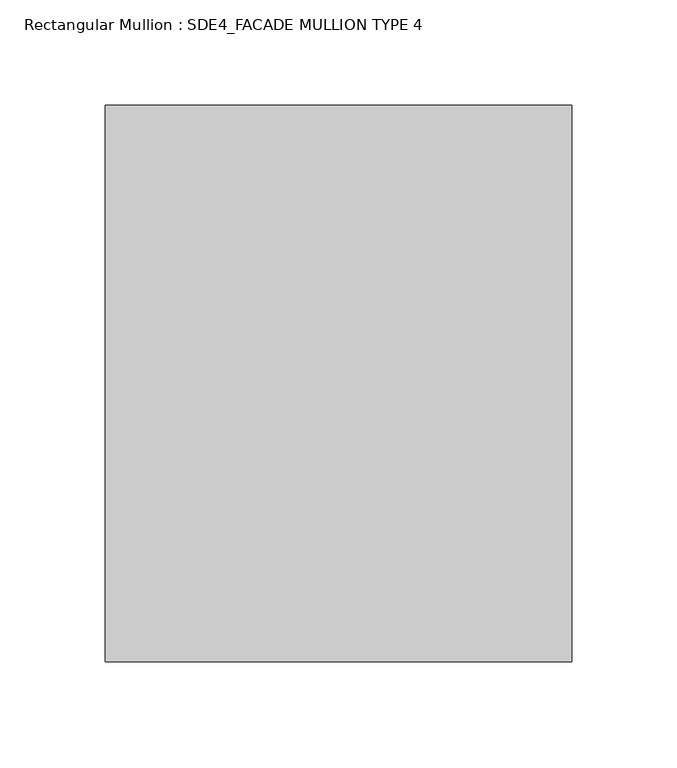
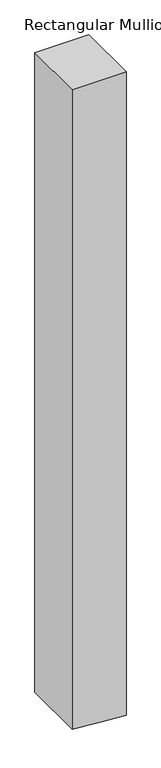
"""IFC4 building model written with IfcOpenShell, lengths in millimetres: member geometry, Rectangular Mullion : SDE4_FACADE MULLION TYPE 4."""

from ifc_helpers import new_model, si_unit, frame, origin, place, context, project, spatial, polyline, outline, extrude, source, transform, mapped, element, save


def rectangular_mullion_sde4_facade_mullion_type_4_16d99790(model_context):
    return source(origin(), model_context, "Body", "SweptSolid", [
        extrude(outline(polyline([(0.0, 111.0), (0.0, -111.0), (-2781.4789383, -111.0), (-2790.2198599, 3.056508), (-2798.4922998, 111.0), (0.0, 111.0)])), frame((0.0, -132.5, 0.0), z_axis=(0.0, 1.0, 0.0), x_axis=(0.0, 0.0, 1.0)), (0.0, 0.0, 1.0), 265.0),
    ])


if __name__ == "__main__":
    model = new_model("IFC4")
    model_context = context("Model", 3, world=origin())
    ifc_project = project(units=[si_unit("LENGTHUNIT", "METRE", prefix="MILLI")], contexts=[model_context])
    site = spatial("IfcSite", under=ifc_project)
    building = spatial("IfcBuilding", under=site)
    placement = place(None, origin())
    rectangular_mullion_sde4_facade_mullion_type_4_shape = rectangular_mullion_sde4_facade_mullion_type_4_16d99790(model_context)
    element("IfcMember", 1, ObjectType="Rectangular Mullion : SDE4_FACADE MULLION TYPE 4", at=placement, inside=building, context=model_context, shape_type="MappedRepresentation", body=[
        mapped(rectangular_mullion_sde4_facade_mullion_type_4_shape, transform((0.0, 0.0, 0.0), x_axis=(1.0, 0.0, 0.0), y_axis=(0.0, 1.0, 0.0), z_axis=(0.0, 0.0, 1.0))),
    ])
    save(model, "model.ifc")

# Revit data of these elements
# Type "Rectangular Mullion : SDE4_FACADE MULLION TYPE 4"
#   built-in parameter 1007322 = 0.869423 (stored number, unit not read)
#   built-in parameter 1007321 = 0.364173 (stored number, unit not read)
#   built-in parameter 1007320 = 0.364173 (stored number, unit not read)
